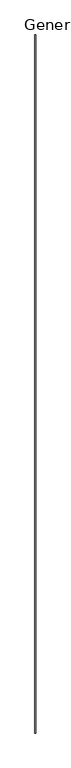
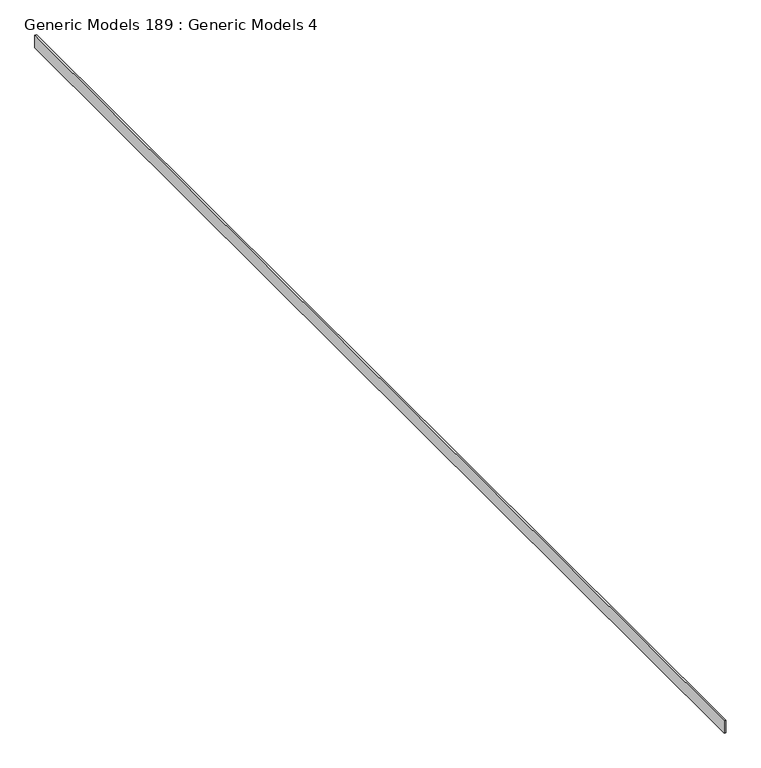
"""IFC4 building model written with IfcOpenShell, lengths in millimetres: proxy geometry, Generic Models 189 : Generic Models 4."""

from ifc_helpers import new_model, si_unit, frame, origin, place, context, project, spatial, polyline, outline, extrude, source, transform, mapped, element, save


def generic_models_189_generic_models_4_30759ed8(model_context):
    return source(origin(), model_context, "Body", "SweptSolid", [
        extrude(outline(polyline([(-6566.4572841, -6864.9230338), (-6585.5072841, -6864.9230338), (-6585.5072841, 7054.2769662), (-6566.4572841, 7054.2769662), (-6566.4572841, -6864.9230338)])), frame((0.0, 0.0, 126345.591095), z_axis=(0.0, 0.0, 1.0), x_axis=(1.0, 0.0, 0.0)), (0.0, 0.0, 1.0), 154.4259718),
    ])


if __name__ == "__main__":
    model = new_model("IFC4")
    model_context = context("Model", 3, world=origin())
    ifc_project = project(units=[si_unit("LENGTHUNIT", "METRE", prefix="MILLI")], contexts=[model_context])
    site = spatial("IfcSite", under=ifc_project)
    building = spatial("IfcBuilding", under=site)
    placement = place(None, origin())
    generic_models_189_generic_models_4_shape = generic_models_189_generic_models_4_30759ed8(model_context)
    element("IfcBuildingElementProxy", 1, Name="Generic Models 189 : Generic Models 4", ObjectType="Generic Models 189 : Generic Models 4", at=placement, inside=building, context=model_context, shape_type="MappedRepresentation", body=[
        mapped(generic_models_189_generic_models_4_shape, transform((0.0, 0.0, 0.0), x_axis=(1.0, 0.0, 0.0), y_axis=(0.0, 1.0, 0.0), z_axis=(0.0, 0.0, 1.0))),
    ])
    save(model, "model.ifc")

# Revit data of these elements
# Element 1 (IfcBuildingElementProxy, "Generic Models 189 : Generic Models 4")
#   Materials on its faces: "_T&G FIRE RETARDANT WOOD SOFFIT O/ BUILDING PAPER"
# Materials
#   "_T&G FIRE RETARDANT WOOD SOFFIT O/ BUILDING PAPER": class "Generic", colour RGB 177 130 114, transparency 0, Cost = 0
